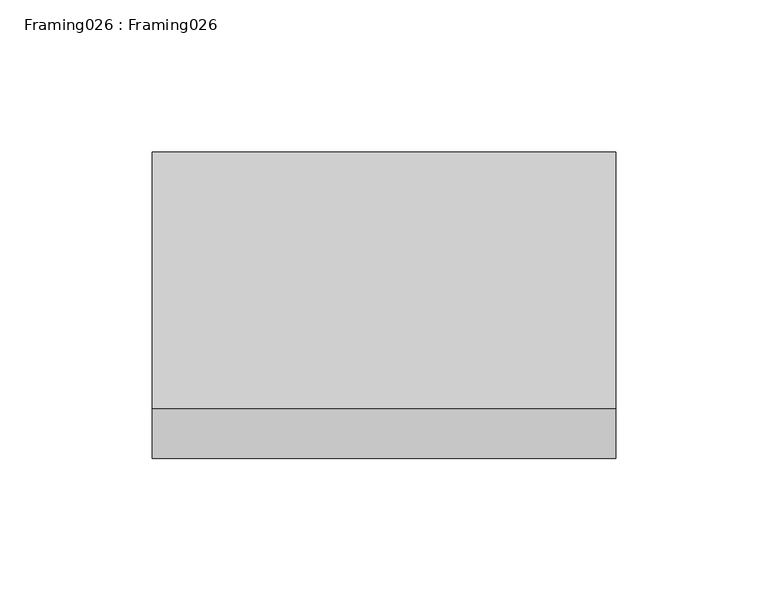
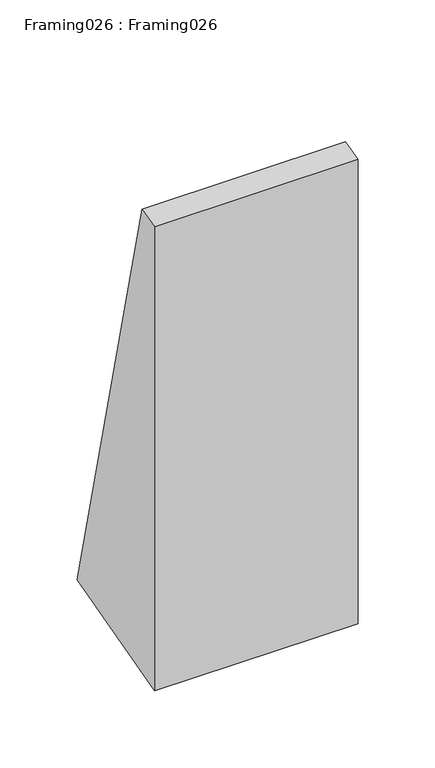
"""IFC4 building model written with IfcOpenShell, lengths in millimetres: proxy geometry, Framing026 : Framing026."""

import ifcopenshell
import ifcopenshell.guid

model = None  # the IFC model being written
_history = None  # IfcOwnerHistory: only IFC2X3 demands one
_inside = {}  # id of a spatial element -> (the spatial element, [elements in it])
_under = {}  # id of a project, library or spatial element -> (it, [spatial elements below it])
_declared = {}  # id of a project -> (the project, [libraries it declares])
_typed = {}  # id of a type object -> (the type object, [elements of that type])
_made_of = {}  # id of a material, layer set ... -> (it, [elements and type objects made of it])


def new_model(schema):
    """Start an empty IFC model of exactly this schema.

    Asked for "IFC4X3", IfcOpenShell would pick the latest addendum, in which some entities
    have other attributes; the version numbers below select the first issue.
    IFC2X3 requires an IfcOwnerHistory on every rooted entity: one is made here for all.
    """
    global model, _history
    if schema == "IFC4X3":
        model = ifcopenshell.file(schema_version=(4, 3, 0, 0))
    else:
        model = ifcopenshell.file(schema=schema)
    _inside.clear()
    _under.clear()
    _declared.clear()
    _typed.clear()
    _made_of.clear()
    _history = None
    if model.schema == "IFC2X3":
        org = make("IfcOrganization", Name="unknown")
        user = make(
            "IfcPersonAndOrganization",
            ThePerson=make("IfcPerson", FamilyName="unknown"),
            TheOrganization=org,
        )
        app = make(
            "IfcApplication",
            ApplicationDeveloper=org,
            Version="unknown",
            ApplicationFullName="unknown",
            ApplicationIdentifier="unknown",
        )
        _history = make(
            "IfcOwnerHistory",
            OwningUser=user,
            OwningApplication=app,
            ChangeAction="ADDED",
            CreationDate=0,
        )
    return model


def make(cls, **values):
    """One entity of the class cls with the attributes given. An attribute that is None is left unset."""
    return model.create_entity(
        cls, **{name: value for name, value in values.items() if value is not None}
    )


def rooted(cls, **values):
    """An entity with a GlobalId (a new one), such as an element, a storey or a relation."""
    return make(cls, GlobalId=ifcopenshell.guid.new(), OwnerHistory=_history, **values)


def si_unit(unit_type, name, prefix=None):
    """IfcSIUnit, for example si_unit("LENGTHUNIT", "METRE", prefix="MILLI")."""
    return make("IfcSIUnit", UnitType=unit_type, Prefix=prefix, Name=name)


def assignment(units):
    """IfcUnitAssignment: the units of a project."""
    return None if units is None else make("IfcUnitAssignment", Units=units)


def point(xyz):
    """IfcCartesianPoint."""
    return None if xyz is None else make("IfcCartesianPoint", Coordinates=xyz)


def direction(xyz):
    """IfcDirection."""
    return None if xyz is None else make("IfcDirection", DirectionRatios=xyz)


def frame(location, z_axis=None, x_axis=None):
    """IfcAxis2Placement3D, a coordinate frame: its origin and axes. An axis left out is left unset."""
    return make(
        "IfcAxis2Placement3D",
        Location=point(location),
        Axis=direction(z_axis),
        RefDirection=direction(x_axis),
    )


def origin():
    """The frame at (0, 0, 0) with its axes left unset."""
    return frame((0.0, 0.0, 0.0))


def place(relative_to, where):
    """IfcLocalPlacement: puts the frame where relative to a parent placement (None: the world)."""
    return make(
        "IfcLocalPlacement", PlacementRelTo=relative_to, RelativePlacement=where
    )


def context(
    kind, dimensions, precision=None, world=None, true_north=None, identifier=None
):
    """IfcGeometricRepresentationContext, for example the 3D "Model" context."""
    return make(
        "IfcGeometricRepresentationContext",
        ContextIdentifier=identifier,
        ContextType=kind,
        CoordinateSpaceDimension=dimensions,
        Precision=precision,
        WorldCoordinateSystem=world,
        TrueNorth=true_north,
    )


def project(units=None, contexts=None):
    """IfcProject with its units and contexts."""
    return rooted(
        "IfcProject",
        Name="project",
        RepresentationContexts=contexts,
        UnitsInContext=assignment(units),
    )


def spatial(cls, under=None, at=None, **own):
    """A site, building, storey or space (cls), placed at a placement, below another one or the project."""
    s = rooted(cls, ObjectPlacement=at, **own)
    if under is not None:
        _under.setdefault(under.id(), (under, []))[1].append(s)
    return s


def polyline(points):
    """IfcPolyline through the points."""
    return make("IfcPolyline", Points=[point(p) for p in points])


def outline(outer, holes=None, kind="AREA"):
    """IfcArbitraryClosedProfileDef: a profile drawn as a closed curve; with holes, ...WithVoids."""
    if holes is None:
        return make("IfcArbitraryClosedProfileDef", ProfileType=kind, OuterCurve=outer)
    return make(
        "IfcArbitraryProfileDefWithVoids",
        ProfileType=kind,
        OuterCurve=outer,
        InnerCurves=holes,
    )


def extrude(swept, where, along, depth):
    """IfcExtrudedAreaSolid: the profile swept, set in the frame where, extruded along a direction by depth."""
    return make(
        "IfcExtrudedAreaSolid",
        SweptArea=swept,
        Position=where,
        ExtrudedDirection=direction(along),
        Depth=depth,
    )


def shape(context_of_items, identifier, shape_type, items):
    """IfcShapeRepresentation: the items that make up one representation, for example the "Body"."""
    return make(
        "IfcShapeRepresentation",
        ContextOfItems=context_of_items,
        RepresentationIdentifier=identifier,
        RepresentationType=shape_type,
        Items=items,
    )


def source(mapping_origin, context_of_items, identifier, shape_type, items):
    """IfcRepresentationMap: a shape defined once, which mapped items show again and again."""
    return make(
        "IfcRepresentationMap",
        MappingOrigin=mapping_origin,
        MappedRepresentation=shape(context_of_items, identifier, shape_type, items),
    )


def transform(
    local_origin,
    x_axis=None,
    y_axis=None,
    z_axis=None,
    scale=None,
    scale2=None,
    scale3=None,
    uniform=True,
):
    """IfcCartesianTransformationOperator3D, or its non-uniform kind. x_axis, y_axis, z_axis: its Axis1, 2, 3."""
    if uniform:
        return make(
            "IfcCartesianTransformationOperator3D",
            Axis1=direction(x_axis),
            Axis2=direction(y_axis),
            LocalOrigin=point(local_origin),
            Scale=scale,
            Axis3=direction(z_axis),
        )
    return make(
        "IfcCartesianTransformationOperator3DnonUniform",
        Axis1=direction(x_axis),
        Axis2=direction(y_axis),
        LocalOrigin=point(local_origin),
        Scale=scale,
        Axis3=direction(z_axis),
        Scale2=scale2,
        Scale3=scale3,
    )


def mapped(mapping_source, mapping_target):
    """IfcMappedItem: shows the shape of a source again, moved by a transform."""
    return make(
        "IfcMappedItem", MappingSource=mapping_source, MappingTarget=mapping_target
    )


def made_of(thing, what):
    """Note that an element or type object is made of a material, layer set ...; save() writes the relation."""
    if what is not None:
        _made_of.setdefault(what.id(), (what, []))[1].append(thing)
    return thing


def element(
    cls,
    number,
    at=None,
    inside=None,
    cuts=None,
    type_object=None,
    material=None,
    context=None,
    identifier="Body",
    shape_type=None,
    held_by="IfcProductDefinitionShape",
    body=None,
    shapes=None,
    **own,
):
    """One element of the class cls, such as IfcWall. Its Tag is "e" and its number.

    at: its placement. inside: the storey or other place that contains it. cuts: it is an
    opening in that element (IfcRelVoidsElement). A single representation is given by context,
    identifier, shape_type and body (its items); several are given by shapes. held_by: the class
    of the entity that holds the representations. save() writes the other relations.
    """
    e = rooted(cls, Tag="e%d" % number, ObjectPlacement=at, **own)
    if body is not None:
        shapes = [shape(context, identifier, shape_type, body)]
    if shapes is not None:
        e.Representation = make(held_by, Representations=shapes)
    if inside is not None:
        _inside.setdefault(inside.id(), (inside, []))[1].append(e)
    if cuts is not None:
        rooted(
            "IfcRelVoidsElement", RelatingBuildingElement=cuts, RelatedOpeningElement=e
        )
    if type_object is not None:
        _typed.setdefault(type_object.id(), (type_object, []))[1].append(e)
    return made_of(e, material)


def aggregate(whole, parts):
    """IfcRelAggregates: a whole, such as a stair, and the parts it consists of."""
    return rooted("IfcRelAggregates", RelatingObject=whole, RelatedObjects=parts)


def save(model, path):
    """Write the relations noted so far, then the file.

    IfcRelAggregates (storeys below a building ...), IfcRelContainedInSpatialStructure (elements
    in a storey), IfcRelDefinesByType, IfcRelAssociatesMaterial and IfcRelDeclares: one each for
    every whole, place, type object, material and project.
    """
    for whole, parts in _under.values():
        aggregate(whole, parts)
    for where, things in _inside.values():
        rooted(
            "IfcRelContainedInSpatialStructure",
            RelatedElements=things,
            RelatingStructure=where,
        )
    for kind, things in _typed.values():
        rooted("IfcRelDefinesByType", RelatedObjects=things, RelatingType=kind)
    for what, things in _made_of.values():
        rooted("IfcRelAssociatesMaterial", RelatedObjects=things, RelatingMaterial=what)
    for by, libraries in _declared.values():
        rooted("IfcRelDeclares", RelatingContext=by, RelatedDefinitions=libraries)
    model.write(path)


def framing026_framing026_72f8b337(model_context):
    return source(origin(), model_context, "Body", "SweptSolid", [
        extrude(outline(polyline([(-5532.4912696, 42724.5605159), (-5447.9743192, 42379.6308633), (-5548.7675368, 42352.8540702), (-5548.7675368, 42720.572397), (-5532.4912696, 42724.5605159)])), frame((12383.0178845, 0.0, 0.0), z_axis=(1.0, 0.0, 0.0), x_axis=(0.0, 1.0, 0.0)), (0.0, 0.0, 1.0), 152.4),
    ])


if __name__ == "__main__":
    model = new_model("IFC4")
    model_context = context("Model", 3, world=origin())
    ifc_project = project(units=[si_unit("LENGTHUNIT", "METRE", prefix="MILLI")], contexts=[model_context])
    site = spatial("IfcSite", under=ifc_project)
    building = spatial("IfcBuilding", under=site)
    placement = place(None, origin())
    framing026_framing026_shape = framing026_framing026_72f8b337(model_context)
    element("IfcBuildingElementProxy", 1, Name="Framing026 : Framing026", ObjectType="Framing026 : Framing026", at=placement, inside=building, context=model_context, shape_type="MappedRepresentation", body=[
        mapped(framing026_framing026_shape, transform((0.0, 0.0, 0.0), x_axis=(1.0, 0.0, 0.0), y_axis=(0.0, 1.0, 0.0), z_axis=(0.0, 0.0, 1.0))),
    ])
    save(model, "model.ifc")

# Revit data of these elements
# Type "Framing026 : Framing026"
#   NameOverride = "Framing026"
# Element 1 (IfcBuildingElementProxy, "Framing026 : Framing026")
#   Materials on its faces: "WOOD FRAMING (SEE STRUCT DWGS)"
# Materials
#   "WOOD FRAMING (SEE STRUCT DWGS)": class "Unassigned", colour RGB 224 188 168, transparency 0, Cost = 0
